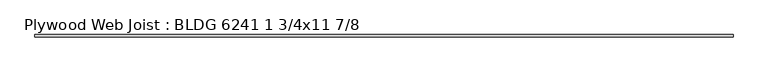
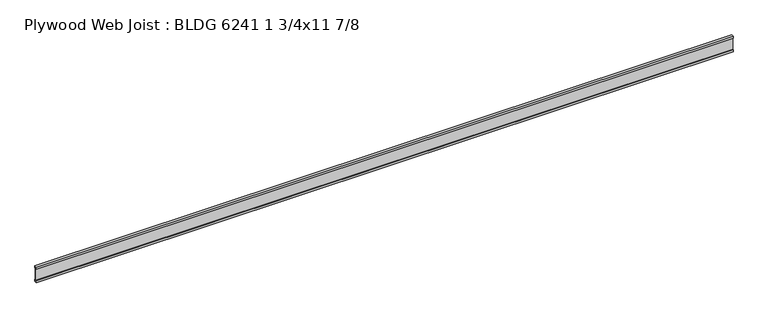
"""IFC4 building model written with IfcOpenShell, lengths in millimetres: beam geometry, Plywood Web Joist : BLDG 6241 1 3/4x11 7/8."""

from ifc_helpers import new_model, si_unit, frame, origin, place, context, project, spatial, polyline, outline, extrude, source, transform, mapped, element, save


def plywood_web_joist_bldg_6241_1_3_4x11_7_8_0dbcbf17(model_context):
    return source(origin(), model_context, "Body", "SweptSolid", [
        extrude(outline(polyline([(-22.225, 150.8125), (22.225, 150.8125), (22.225, 112.7125), (4.7625, 112.7125), (4.7625, 119.0625), (-4.7625, 119.0625), (-4.7625, 112.7125), (-22.225, 112.7125), (-22.225, 150.8125)])), frame((-6365.875, 0.0, 0.0), z_axis=(1.0, 0.0, 0.0), x_axis=(0.0, 1.0, 0.0)), (0.0, 0.0, 1.0), 12731.75),
        extrude(outline(polyline([(22.225, -112.7125), (22.225, -150.8125), (-22.225, -150.8125), (-22.225, -112.7125), (-4.7625, -112.7125), (-4.7625, -118.3285374), (4.7625, -118.3285374), (4.7625, -112.7125), (22.225, -112.7125)])), frame((-6365.875, 0.0, 0.0), z_axis=(1.0, 0.0, 0.0), x_axis=(0.0, 1.0, 0.0)), (0.0, 0.0, 1.0), 12731.75),
        extrude(outline(polyline([(6365.875, 4.7625), (6365.875, -4.7625), (-6365.875, -4.7625), (-6365.875, 4.7625), (6365.875, 4.7625)])), frame((0.0, 0.0, -118.3285374), z_axis=(0.0, 0.0, 1.0), x_axis=(1.0, 0.0, 0.0)), (0.0, 0.0, 1.0), 237.3910374),
    ])


if __name__ == "__main__":
    model = new_model("IFC4")
    model_context = context("Model", 3, world=origin())
    ifc_project = project(units=[si_unit("LENGTHUNIT", "METRE", prefix="MILLI")], contexts=[model_context])
    site = spatial("IfcSite", under=ifc_project)
    building = spatial("IfcBuilding", under=site)
    placement = place(None, origin())
    plywood_web_joist_bldg_6241_1_3_4x11_7_8_shape = plywood_web_joist_bldg_6241_1_3_4x11_7_8_0dbcbf17(model_context)
    element("IfcBeam", 1, ObjectType="Plywood Web Joist : BLDG 6241 1 3/4x11 7/8", at=placement, inside=building, context=model_context, shape_type="MappedRepresentation", body=[
        mapped(plywood_web_joist_bldg_6241_1_3_4x11_7_8_shape, transform((0.0, 0.0, 0.0), x_axis=(1.0, 0.0, 0.0), y_axis=(0.0, 1.0, 0.0), z_axis=(0.0, 0.0, 1.0))),
    ])
    save(model, "model.ifc")

# Revit data of these elements
# Type "Plywood Web Joist : BLDG 6241 1 3/4x11 7/8"
#   Assembly Code = "B10"
#   Length [instance default] = 5' - 0"
#   b = 0' - 1 3/4"
#   d = 0' - 11 7/8"
#   Structural Material [instance default] = Softwood, Lumber
# Element 1 (IfcBeam, "Plywood Web Joist : BLDG 6241 1 3/4x11 7/8")
#   Materials on its faces: "Softwood, Lumber"
# Materials
#   "Softwood, Lumber": class "Wood", colour RGB 223 192 134, transparency 0, Description = "Pinus Echinata", Cost = 0
